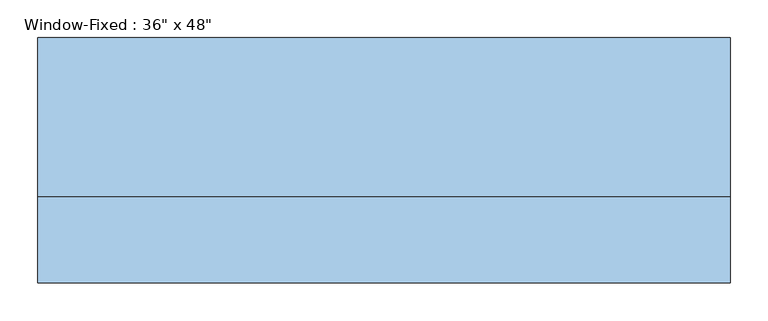
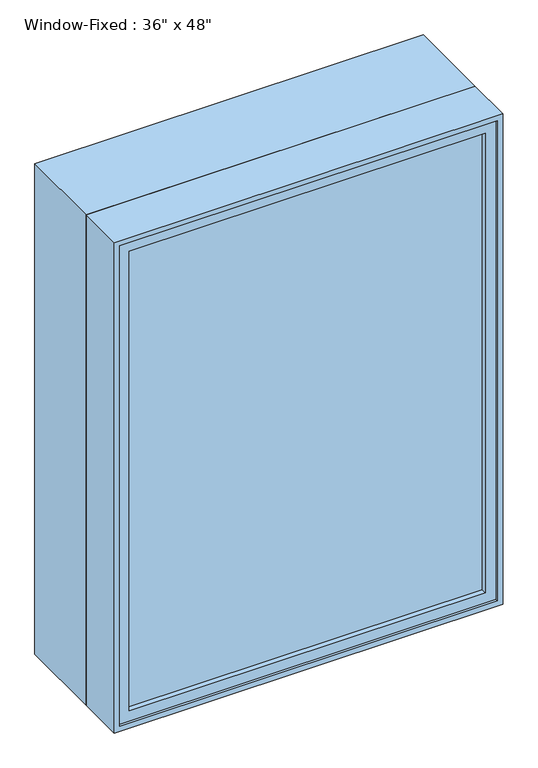
"""IFC4 building model written with IfcOpenShell, lengths in millimetres: window geometry."""

from ifc_helpers import new_model, si_unit, frame, origin, place, context, project, spatial, polyline, outline, extrude, faceted_brep, source, transform, mapped, element, save


def window_ebfb4af0(model_context):
    return source(origin(), model_context, "Body", "SolidModel", [
        extrude(outline(polyline([(419.1, -152.4), (-419.1, -152.4), (-419.1, -146.05), (419.1, -146.05), (419.1, -152.4)])), frame((0.0, 0.0, 952.5), z_axis=(0.0, 0.0, 1.0), x_axis=(1.0, 0.0, 0.0)), (0.0, 0.0, 1.0), 1143.0),
        extrude(outline(polyline([(-419.1, -133.35), (419.1, -133.35), (419.1, -139.7), (-419.1, -139.7), (-419.1, -133.35)])), frame((0.0, 0.0, 952.5), z_axis=(0.0, 0.0, 1.0), x_axis=(1.0, 0.0, 0.0)), (0.0, 0.0, 1.0), 1143.0),
        extrude(outline(polyline([(927.1, -444.5), (927.1, 444.5), (2120.9, 444.5), (2120.9, -444.5), (927.1, -444.5)]), holes=[polyline([(952.5, 419.1), (952.5, -419.1), (2095.5, -419.1), (2095.5, 419.1), (952.5, 419.1)])]), frame((0.0, -165.1, 0.0), z_axis=(0.0, 1.0, 0.0), x_axis=(0.0, 0.0, 1.0)), (0.0, 0.0, 1.0), 44.45),
        extrude(outline(polyline([(2133.6, -457.2), (914.4, -457.2), (914.4, 457.2), (2133.6, 457.2), (2133.6, -457.2)]), holes=[polyline([(2120.9, 444.5), (927.1, 444.5), (927.1, -444.5), (2120.9, -444.5), (2120.9, 444.5)])]), frame((0.0, -57.15, 0.0), z_axis=(0.0, 1.0, 0.0), x_axis=(0.0, 0.0, 1.0)), (0.0, 0.0, 1.0), 209.55),
        faceted_brep([(457.2, -57.15, 2133.6), (-457.2, -57.15, 2133.6), (-457.2, -171.45, 2133.6), (457.2, -171.45, 2133.6), (-457.2, -57.15, 914.4), (-457.2, -171.45, 914.4), (457.2, -57.15, 914.4), (457.2, -171.45, 914.4), (425.45, -57.15, 2101.85), (-425.45, -57.15, 2101.85), (-425.45, -57.15, 946.15), (425.45, -57.15, 946.15), (-444.5, -171.45, 2120.9), (444.5, -171.45, 2120.9), (444.5, -171.45, 927.1), (-444.5, -171.45, 927.1), (425.45, -120.65, 2101.85), (-425.45, -120.65, 2101.85), (-444.5, -120.65, 2120.9), (444.5, -120.65, 2120.9), (-425.45, -120.65, 946.15), (-444.5, -120.65, 927.1), (425.45, -120.65, 946.15), (444.5, -120.65, 927.1)], [[[0, 1, 2, 3]], [[1, 4, 5, 2]], [[4, 6, 7, 5]], [[1, 0, 6, 4], [8, 9, 10, 11]], [[6, 0, 3, 7]], [[3, 2, 5, 7], [12, 13, 14, 15]], [[16, 17, 9, 8]], [[13, 12, 18, 19]], [[17, 20, 10, 9]], [[12, 15, 21, 18]], [[20, 22, 11, 10]], [[15, 14, 23, 21]], [[22, 16, 8, 11]], [[19, 18, 21, 23], [17, 16, 22, 20]], [[14, 13, 19, 23]]]),
    ])


if __name__ == "__main__":
    model = new_model("IFC4")
    model_context = context("Model", 3, world=origin())
    ifc_project = project(units=[si_unit("LENGTHUNIT", "METRE", prefix="MILLI")], contexts=[model_context])
    site = spatial("IfcSite", under=ifc_project)
    building = spatial("IfcBuilding", under=site)
    placement = place(None, origin())
    window_shape = window_ebfb4af0(model_context)
    element("IfcWindow", 1, ObjectType="Window-Fixed : 36\" x 48\"", at=placement, inside=building, context=model_context, shape_type="MappedRepresentation", body=[
        mapped(window_shape, transform((0.0, 0.0, 0.0), x_axis=(1.0, 0.0, 0.0), y_axis=(0.0, 1.0, 0.0), z_axis=(0.0, 0.0, 1.0))),
    ])
    save(model, "model.ifc")

# Revit data of these elements
# Type "Window-Fixed : 36\" x 48\""
#   Type Mark = "H"
#   Fire Rating = "0.5h"
#   Assembly Code = "B2020100"
#   Analytic Construction = "Double glazing - domestic"
#   Window Inset [instance default] = 0' - 0"
#   Wall Thickness [instance default] = 0' - 6"
#   Visual Light Transmittance = 0.81
#   Thermal Resistance (R) = 1.8146 (h·ft²·°F)/BTU
#   Solar Heat Gain Coefficient = 0.76
#   Rough Width = 3' - 0 1/2"
#   Rough Height = 4' - 0 1/2"
#   Interior Wall Closure [instance default] = 0' - 2 1/4"
#   Height = 4' - 0"
#   Heat Transfer Coefficient (U) = 0.5511 BTU/(h·ft²·°F)
#   Frame Extension [instance default] = 0' - 0 1/4"
#   Exterior Wall Closure [instance default] = 0' - 1 1/4"
#   Extension Jamb [instance default] = 0' - 2 1/4"
#   Default Sill Height = 3' - 0"
#   Width = 3' - 0"
#   Muntin Visibility = yes
#   Interior Trim Visibility [instance default] = yes
#   Exterior Trim Visibility [instance default] = yes
#   Extension Jamb Visibility [instance default] = yes
#   Muntin Pattern = Muntin Pattern_2x2 : Muntin Pattern_2x2
#   Interior Trim Material = Wood - Stained
#   Interior Trim = Trim-Window-Interior-Flat : Picture Frame
#   Interior Frame Material = Wood - Stained
#   Glass Panel Material = Glass
#   Exterior Trim Material = Clad - White
#   Exterior Trim = Trim-Window-Exterior-Flat : with Sill
#   Exterior Frame Material = Clad - White
#   Wall Closure = (empty or 0)
# Element 1 (IfcWindow, "Window-Fixed : 36\" x 48\"")
#   Wall Thickness = 1' - 0"
#   Extension Jamb = 0' - 8 1/4"
#   Materials on its faces: "Wood - Stained", "Glass", "Clad - White"
# Materials
#   "Wood - Stained": class "Wood", colour RGB 224 178 126, transparency 0, Cost = 0
#   "Glass": class "Unassigned", colour RGB 0 128 192, transparency 0.75, Description = "Glass"
#   "Clad - White": class "Wood", colour RGB 242 242 238, transparency 0, Cost = 0
